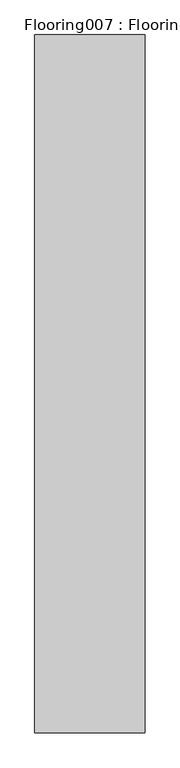
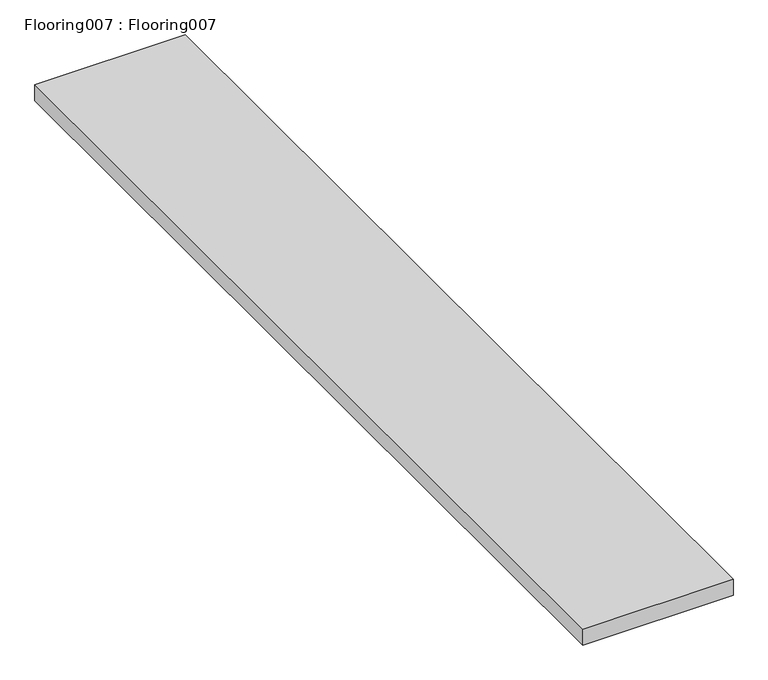
"""IFC4 building model written with IfcOpenShell, lengths in millimetres: proxy geometry, Flooring007 : Flooring007."""

from ifc_helpers import new_model, si_unit, frame, origin, place, context, project, spatial, polyline, outline, extrude, source, transform, mapped, element, save


def flooring007_flooring007_d512611b(model_context):
    return source(origin(), model_context, "Body", "SweptSolid", [
        extrude(outline(polyline([(-9437.1459961, 7982.1531721), (-9753.753418, 7982.1531721), (-9753.753418, 9982.1531721), (-9437.1459961, 9982.1531721), (-9437.1459961, 7982.1531721)])), frame((0.0, 0.0, 40127.7030395), z_axis=(0.0, 0.0, 1.0), x_axis=(1.0, 0.0, 0.0)), (0.0, 0.0, 1.0), 35.7929688),
    ])


if __name__ == "__main__":
    model = new_model("IFC4")
    model_context = context("Model", 3, world=origin())
    ifc_project = project(units=[si_unit("LENGTHUNIT", "METRE", prefix="MILLI")], contexts=[model_context])
    site = spatial("IfcSite", under=ifc_project)
    building = spatial("IfcBuilding", under=site)
    placement = place(None, origin())
    flooring007_flooring007_shape = flooring007_flooring007_d512611b(model_context)
    element("IfcBuildingElementProxy", 1, Name="Flooring007 : Flooring007", ObjectType="Flooring007 : Flooring007", at=placement, inside=building, context=model_context, shape_type="MappedRepresentation", body=[
        mapped(flooring007_flooring007_shape, transform((0.0, 0.0, 0.0), x_axis=(1.0, 0.0, 0.0), y_axis=(0.0, 1.0, 0.0), z_axis=(0.0, 0.0, 1.0))),
    ])
    save(model, "model.ifc")

# Revit data of these elements
# Type "Flooring007 : Flooring007"
#   NameOverride = "Flooring007"
# Element 1 (IfcBuildingElementProxy, "Flooring007 : Flooring007")
#   Materials on its faces: "TERRACE FLOORING TBD"
# Materials
#   "TERRACE FLOORING TBD": class "Unassigned", colour RGB 128 128 128, transparency 0
